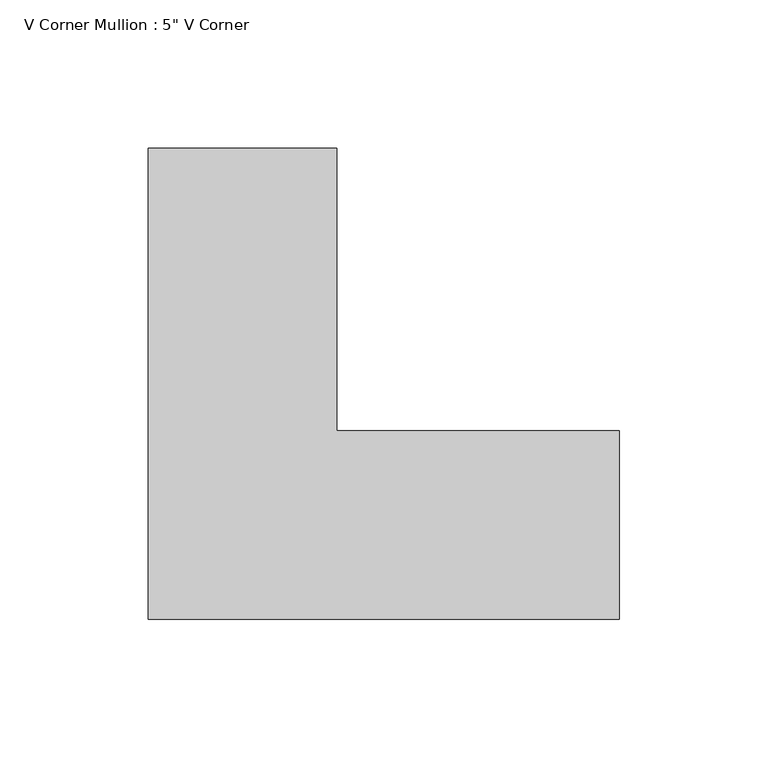
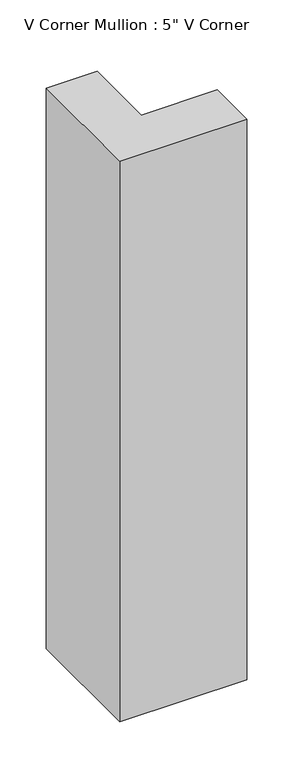
"""IFC4 building model written with IfcOpenShell, lengths in millimetres: member geometry."""

import ifcopenshell
import ifcopenshell.guid

model = None  # the IFC model being written
_history = None  # IfcOwnerHistory: only IFC2X3 demands one
_inside = {}  # id of a spatial element -> (the spatial element, [elements in it])
_under = {}  # id of a project, library or spatial element -> (it, [spatial elements below it])
_declared = {}  # id of a project -> (the project, [libraries it declares])
_typed = {}  # id of a type object -> (the type object, [elements of that type])
_made_of = {}  # id of a material, layer set ... -> (it, [elements and type objects made of it])


def new_model(schema):
    """Start an empty IFC model of exactly this schema.

    Asked for "IFC4X3", IfcOpenShell would pick the latest addendum, in which some entities
    have other attributes; the version numbers below select the first issue.
    IFC2X3 requires an IfcOwnerHistory on every rooted entity: one is made here for all.
    """
    global model, _history
    if schema == "IFC4X3":
        model = ifcopenshell.file(schema_version=(4, 3, 0, 0))
    else:
        model = ifcopenshell.file(schema=schema)
    _inside.clear()
    _under.clear()
    _declared.clear()
    _typed.clear()
    _made_of.clear()
    _history = None
    if model.schema == "IFC2X3":
        org = make("IfcOrganization", Name="unknown")
        user = make(
            "IfcPersonAndOrganization",
            ThePerson=make("IfcPerson", FamilyName="unknown"),
            TheOrganization=org,
        )
        app = make(
            "IfcApplication",
            ApplicationDeveloper=org,
            Version="unknown",
            ApplicationFullName="unknown",
            ApplicationIdentifier="unknown",
        )
        _history = make(
            "IfcOwnerHistory",
            OwningUser=user,
            OwningApplication=app,
            ChangeAction="ADDED",
            CreationDate=0,
        )
    return model


def make(cls, **values):
    """One entity of the class cls with the attributes given. An attribute that is None is left unset."""
    return model.create_entity(
        cls, **{name: value for name, value in values.items() if value is not None}
    )


def rooted(cls, **values):
    """An entity with a GlobalId (a new one), such as an element, a storey or a relation."""
    return make(cls, GlobalId=ifcopenshell.guid.new(), OwnerHistory=_history, **values)


def si_unit(unit_type, name, prefix=None):
    """IfcSIUnit, for example si_unit("LENGTHUNIT", "METRE", prefix="MILLI")."""
    return make("IfcSIUnit", UnitType=unit_type, Prefix=prefix, Name=name)


def assignment(units):
    """IfcUnitAssignment: the units of a project."""
    return None if units is None else make("IfcUnitAssignment", Units=units)


def point(xyz):
    """IfcCartesianPoint."""
    return None if xyz is None else make("IfcCartesianPoint", Coordinates=xyz)


def direction(xyz):
    """IfcDirection."""
    return None if xyz is None else make("IfcDirection", DirectionRatios=xyz)


def frame(location, z_axis=None, x_axis=None):
    """IfcAxis2Placement3D, a coordinate frame: its origin and axes. An axis left out is left unset."""
    return make(
        "IfcAxis2Placement3D",
        Location=point(location),
        Axis=direction(z_axis),
        RefDirection=direction(x_axis),
    )


def origin():
    """The frame at (0, 0, 0) with its axes left unset."""
    return frame((0.0, 0.0, 0.0))


def place(relative_to, where):
    """IfcLocalPlacement: puts the frame where relative to a parent placement (None: the world)."""
    return make(
        "IfcLocalPlacement", PlacementRelTo=relative_to, RelativePlacement=where
    )


def context(
    kind, dimensions, precision=None, world=None, true_north=None, identifier=None
):
    """IfcGeometricRepresentationContext, for example the 3D "Model" context."""
    return make(
        "IfcGeometricRepresentationContext",
        ContextIdentifier=identifier,
        ContextType=kind,
        CoordinateSpaceDimension=dimensions,
        Precision=precision,
        WorldCoordinateSystem=world,
        TrueNorth=true_north,
    )


def project(units=None, contexts=None):
    """IfcProject with its units and contexts."""
    return rooted(
        "IfcProject",
        Name="project",
        RepresentationContexts=contexts,
        UnitsInContext=assignment(units),
    )


def spatial(cls, under=None, at=None, **own):
    """A site, building, storey or space (cls), placed at a placement, below another one or the project."""
    s = rooted(cls, ObjectPlacement=at, **own)
    if under is not None:
        _under.setdefault(under.id(), (under, []))[1].append(s)
    return s


def polyline(points):
    """IfcPolyline through the points."""
    return make("IfcPolyline", Points=[point(p) for p in points])


def outline(outer, holes=None, kind="AREA"):
    """IfcArbitraryClosedProfileDef: a profile drawn as a closed curve; with holes, ...WithVoids."""
    if holes is None:
        return make("IfcArbitraryClosedProfileDef", ProfileType=kind, OuterCurve=outer)
    return make(
        "IfcArbitraryProfileDefWithVoids",
        ProfileType=kind,
        OuterCurve=outer,
        InnerCurves=holes,
    )


def extrude(swept, where, along, depth):
    """IfcExtrudedAreaSolid: the profile swept, set in the frame where, extruded along a direction by depth."""
    return make(
        "IfcExtrudedAreaSolid",
        SweptArea=swept,
        Position=where,
        ExtrudedDirection=direction(along),
        Depth=depth,
    )


def shape(context_of_items, identifier, shape_type, items):
    """IfcShapeRepresentation: the items that make up one representation, for example the "Body"."""
    return make(
        "IfcShapeRepresentation",
        ContextOfItems=context_of_items,
        RepresentationIdentifier=identifier,
        RepresentationType=shape_type,
        Items=items,
    )


def source(mapping_origin, context_of_items, identifier, shape_type, items):
    """IfcRepresentationMap: a shape defined once, which mapped items show again and again."""
    return make(
        "IfcRepresentationMap",
        MappingOrigin=mapping_origin,
        MappedRepresentation=shape(context_of_items, identifier, shape_type, items),
    )


def transform(
    local_origin,
    x_axis=None,
    y_axis=None,
    z_axis=None,
    scale=None,
    scale2=None,
    scale3=None,
    uniform=True,
):
    """IfcCartesianTransformationOperator3D, or its non-uniform kind. x_axis, y_axis, z_axis: its Axis1, 2, 3."""
    if uniform:
        return make(
            "IfcCartesianTransformationOperator3D",
            Axis1=direction(x_axis),
            Axis2=direction(y_axis),
            LocalOrigin=point(local_origin),
            Scale=scale,
            Axis3=direction(z_axis),
        )
    return make(
        "IfcCartesianTransformationOperator3DnonUniform",
        Axis1=direction(x_axis),
        Axis2=direction(y_axis),
        LocalOrigin=point(local_origin),
        Scale=scale,
        Axis3=direction(z_axis),
        Scale2=scale2,
        Scale3=scale3,
    )


def mapped(mapping_source, mapping_target):
    """IfcMappedItem: shows the shape of a source again, moved by a transform."""
    return make(
        "IfcMappedItem", MappingSource=mapping_source, MappingTarget=mapping_target
    )


def made_of(thing, what):
    """Note that an element or type object is made of a material, layer set ...; save() writes the relation."""
    if what is not None:
        _made_of.setdefault(what.id(), (what, []))[1].append(thing)
    return thing


def element(
    cls,
    number,
    at=None,
    inside=None,
    cuts=None,
    type_object=None,
    material=None,
    context=None,
    identifier="Body",
    shape_type=None,
    held_by="IfcProductDefinitionShape",
    body=None,
    shapes=None,
    **own,
):
    """One element of the class cls, such as IfcWall. Its Tag is "e" and its number.

    at: its placement. inside: the storey or other place that contains it. cuts: it is an
    opening in that element (IfcRelVoidsElement). A single representation is given by context,
    identifier, shape_type and body (its items); several are given by shapes. held_by: the class
    of the entity that holds the representations. save() writes the other relations.
    """
    e = rooted(cls, Tag="e%d" % number, ObjectPlacement=at, **own)
    if body is not None:
        shapes = [shape(context, identifier, shape_type, body)]
    if shapes is not None:
        e.Representation = make(held_by, Representations=shapes)
    if inside is not None:
        _inside.setdefault(inside.id(), (inside, []))[1].append(e)
    if cuts is not None:
        rooted(
            "IfcRelVoidsElement", RelatingBuildingElement=cuts, RelatedOpeningElement=e
        )
    if type_object is not None:
        _typed.setdefault(type_object.id(), (type_object, []))[1].append(e)
    return made_of(e, material)


def aggregate(whole, parts):
    """IfcRelAggregates: a whole, such as a stair, and the parts it consists of."""
    return rooted("IfcRelAggregates", RelatingObject=whole, RelatedObjects=parts)


def save(model, path):
    """Write the relations noted so far, then the file.

    IfcRelAggregates (storeys below a building ...), IfcRelContainedInSpatialStructure (elements
    in a storey), IfcRelDefinesByType, IfcRelAssociatesMaterial and IfcRelDeclares: one each for
    every whole, place, type object, material and project.
    """
    for whole, parts in _under.values():
        aggregate(whole, parts)
    for where, things in _inside.values():
        rooted(
            "IfcRelContainedInSpatialStructure",
            RelatedElements=things,
            RelatingStructure=where,
        )
    for kind, things in _typed.values():
        rooted("IfcRelDefinesByType", RelatedObjects=things, RelatingType=kind)
    for what, things in _made_of.values():
        rooted("IfcRelAssociatesMaterial", RelatedObjects=things, RelatingMaterial=what)
    for by, libraries in _declared.values():
        rooted("IfcRelDeclares", RelatingContext=by, RelatedDefinitions=libraries)
    model.write(path)


def member_73470b54(model_context):
    return source(origin(), model_context, "Body", "SweptSolid", [
        extrude(outline(polyline([(63.5, -95.25), (-95.25, -95.25), (-95.25, 63.5), (-31.75, 63.5), (-31.75, -31.75), (63.5, -31.75), (63.5, -95.25)])), frame((0.0, 0.0, -740.1977813), z_axis=(0.0, 0.0, 1.0), x_axis=(1.0, 0.0, 0.0)), (0.0, 0.0, 1.0), 740.1977813),
    ])


if __name__ == "__main__":
    model = new_model("IFC4")
    model_context = context("Model", 3, world=origin())
    ifc_project = project(units=[si_unit("LENGTHUNIT", "METRE", prefix="MILLI")], contexts=[model_context])
    site = spatial("IfcSite", under=ifc_project)
    building = spatial("IfcBuilding", under=site)
    placement = place(None, origin())
    member_shape = member_73470b54(model_context)
    element("IfcMember", 1, ObjectType="V Corner Mullion : 5\" V Corner", at=placement, inside=building, context=model_context, shape_type="MappedRepresentation", body=[
        mapped(member_shape, transform((0.0, 0.0, 0.0), x_axis=(1.0, 0.0, 0.0), y_axis=(0.0, 1.0, 0.0), z_axis=(0.0, 0.0, 1.0))),
    ])
    save(model, "model.ifc")

# Revit data of these elements
# Type "V Corner Mullion : 5\" V Corner"
#   built-in parameter 1007355 = 0.416667 (stored number, unit not read)
#   built-in parameter 1007354 = 0.416667 (stored number, unit not read)
#   built-in parameter 1007304 = 0.208333 (stored number, unit not read)
# Element 1 (IfcMember, "V Corner Mullion : 5\" V Corner")
#   Materials on its faces: "Aluminum"
# Materials
#   "Aluminum": class "Metal", colour RGB 247 247 247, transparency 0, Description = "Aluminum 6061", Cost = 0
